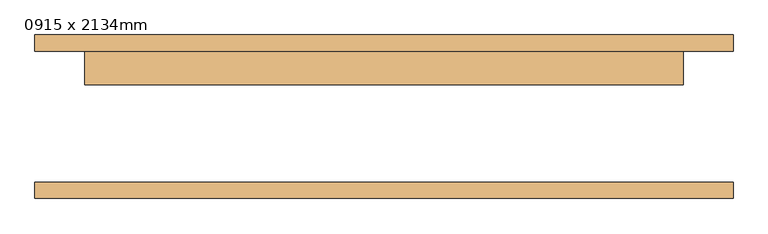
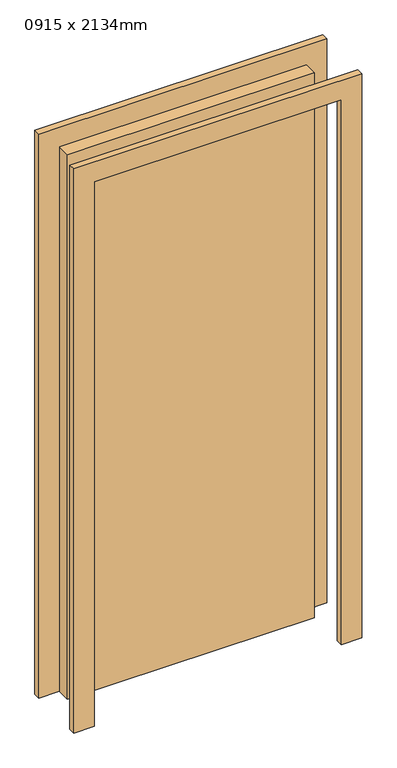
"""IFC4 building model written with IfcOpenShell, lengths in millimetres: door geometry, M_Folha única : 0915 x 2134mm."""

import ifcopenshell
import ifcopenshell.guid

model = None  # the IFC model being written
_history = None  # IfcOwnerHistory: only IFC2X3 demands one
_inside = {}  # id of a spatial element -> (the spatial element, [elements in it])
_under = {}  # id of a project, library or spatial element -> (it, [spatial elements below it])
_declared = {}  # id of a project -> (the project, [libraries it declares])
_typed = {}  # id of a type object -> (the type object, [elements of that type])
_made_of = {}  # id of a material, layer set ... -> (it, [elements and type objects made of it])


def new_model(schema):
    """Start an empty IFC model of exactly this schema.

    Asked for "IFC4X3", IfcOpenShell would pick the latest addendum, in which some entities
    have other attributes; the version numbers below select the first issue.
    IFC2X3 requires an IfcOwnerHistory on every rooted entity: one is made here for all.
    """
    global model, _history
    if schema == "IFC4X3":
        model = ifcopenshell.file(schema_version=(4, 3, 0, 0))
    else:
        model = ifcopenshell.file(schema=schema)
    _inside.clear()
    _under.clear()
    _declared.clear()
    _typed.clear()
    _made_of.clear()
    _history = None
    if model.schema == "IFC2X3":
        org = make("IfcOrganization", Name="unknown")
        user = make(
            "IfcPersonAndOrganization",
            ThePerson=make("IfcPerson", FamilyName="unknown"),
            TheOrganization=org,
        )
        app = make(
            "IfcApplication",
            ApplicationDeveloper=org,
            Version="unknown",
            ApplicationFullName="unknown",
            ApplicationIdentifier="unknown",
        )
        _history = make(
            "IfcOwnerHistory",
            OwningUser=user,
            OwningApplication=app,
            ChangeAction="ADDED",
            CreationDate=0,
        )
    return model


def make(cls, **values):
    """One entity of the class cls with the attributes given. An attribute that is None is left unset."""
    return model.create_entity(
        cls, **{name: value for name, value in values.items() if value is not None}
    )


def rooted(cls, **values):
    """An entity with a GlobalId (a new one), such as an element, a storey or a relation."""
    return make(cls, GlobalId=ifcopenshell.guid.new(), OwnerHistory=_history, **values)


def si_unit(unit_type, name, prefix=None):
    """IfcSIUnit, for example si_unit("LENGTHUNIT", "METRE", prefix="MILLI")."""
    return make("IfcSIUnit", UnitType=unit_type, Prefix=prefix, Name=name)


def assignment(units):
    """IfcUnitAssignment: the units of a project."""
    return None if units is None else make("IfcUnitAssignment", Units=units)


def point(xyz):
    """IfcCartesianPoint."""
    return None if xyz is None else make("IfcCartesianPoint", Coordinates=xyz)


def direction(xyz):
    """IfcDirection."""
    return None if xyz is None else make("IfcDirection", DirectionRatios=xyz)


def frame(location, z_axis=None, x_axis=None):
    """IfcAxis2Placement3D, a coordinate frame: its origin and axes. An axis left out is left unset."""
    return make(
        "IfcAxis2Placement3D",
        Location=point(location),
        Axis=direction(z_axis),
        RefDirection=direction(x_axis),
    )


def origin():
    """The frame at (0, 0, 0) with its axes left unset."""
    return frame((0.0, 0.0, 0.0))


def origin_with_axes():
    """The frame at (0, 0, 0) with the z axis (0, 0, 1) and the x axis (1, 0, 0) written out."""
    return frame((0.0, 0.0, 0.0), z_axis=(0.0, 0.0, 1.0), x_axis=(1.0, 0.0, 0.0))


def place(relative_to, where):
    """IfcLocalPlacement: puts the frame where relative to a parent placement (None: the world)."""
    return make(
        "IfcLocalPlacement", PlacementRelTo=relative_to, RelativePlacement=where
    )


def context(
    kind, dimensions, precision=None, world=None, true_north=None, identifier=None
):
    """IfcGeometricRepresentationContext, for example the 3D "Model" context."""
    return make(
        "IfcGeometricRepresentationContext",
        ContextIdentifier=identifier,
        ContextType=kind,
        CoordinateSpaceDimension=dimensions,
        Precision=precision,
        WorldCoordinateSystem=world,
        TrueNorth=true_north,
    )


def project(units=None, contexts=None):
    """IfcProject with its units and contexts."""
    return rooted(
        "IfcProject",
        Name="project",
        RepresentationContexts=contexts,
        UnitsInContext=assignment(units),
    )


def spatial(cls, under=None, at=None, **own):
    """A site, building, storey or space (cls), placed at a placement, below another one or the project."""
    s = rooted(cls, ObjectPlacement=at, **own)
    if under is not None:
        _under.setdefault(under.id(), (under, []))[1].append(s)
    return s


def polyline(points):
    """IfcPolyline through the points."""
    return make("IfcPolyline", Points=[point(p) for p in points])


def outline(outer, holes=None, kind="AREA"):
    """IfcArbitraryClosedProfileDef: a profile drawn as a closed curve; with holes, ...WithVoids."""
    if holes is None:
        return make("IfcArbitraryClosedProfileDef", ProfileType=kind, OuterCurve=outer)
    return make(
        "IfcArbitraryProfileDefWithVoids",
        ProfileType=kind,
        OuterCurve=outer,
        InnerCurves=holes,
    )


def extrude(swept, where, along, depth):
    """IfcExtrudedAreaSolid: the profile swept, set in the frame where, extruded along a direction by depth."""
    return make(
        "IfcExtrudedAreaSolid",
        SweptArea=swept,
        Position=where,
        ExtrudedDirection=direction(along),
        Depth=depth,
    )


def shape(context_of_items, identifier, shape_type, items):
    """IfcShapeRepresentation: the items that make up one representation, for example the "Body"."""
    return make(
        "IfcShapeRepresentation",
        ContextOfItems=context_of_items,
        RepresentationIdentifier=identifier,
        RepresentationType=shape_type,
        Items=items,
    )


def source(mapping_origin, context_of_items, identifier, shape_type, items):
    """IfcRepresentationMap: a shape defined once, which mapped items show again and again."""
    return make(
        "IfcRepresentationMap",
        MappingOrigin=mapping_origin,
        MappedRepresentation=shape(context_of_items, identifier, shape_type, items),
    )


def transform(
    local_origin,
    x_axis=None,
    y_axis=None,
    z_axis=None,
    scale=None,
    scale2=None,
    scale3=None,
    uniform=True,
):
    """IfcCartesianTransformationOperator3D, or its non-uniform kind. x_axis, y_axis, z_axis: its Axis1, 2, 3."""
    if uniform:
        return make(
            "IfcCartesianTransformationOperator3D",
            Axis1=direction(x_axis),
            Axis2=direction(y_axis),
            LocalOrigin=point(local_origin),
            Scale=scale,
            Axis3=direction(z_axis),
        )
    return make(
        "IfcCartesianTransformationOperator3DnonUniform",
        Axis1=direction(x_axis),
        Axis2=direction(y_axis),
        LocalOrigin=point(local_origin),
        Scale=scale,
        Axis3=direction(z_axis),
        Scale2=scale2,
        Scale3=scale3,
    )


def mapped(mapping_source, mapping_target):
    """IfcMappedItem: shows the shape of a source again, moved by a transform."""
    return make(
        "IfcMappedItem", MappingSource=mapping_source, MappingTarget=mapping_target
    )


def made_of(thing, what):
    """Note that an element or type object is made of a material, layer set ...; save() writes the relation."""
    if what is not None:
        _made_of.setdefault(what.id(), (what, []))[1].append(thing)
    return thing


def element(
    cls,
    number,
    at=None,
    inside=None,
    cuts=None,
    type_object=None,
    material=None,
    context=None,
    identifier="Body",
    shape_type=None,
    held_by="IfcProductDefinitionShape",
    body=None,
    shapes=None,
    **own,
):
    """One element of the class cls, such as IfcWall. Its Tag is "e" and its number.

    at: its placement. inside: the storey or other place that contains it. cuts: it is an
    opening in that element (IfcRelVoidsElement). A single representation is given by context,
    identifier, shape_type and body (its items); several are given by shapes. held_by: the class
    of the entity that holds the representations. save() writes the other relations.
    """
    e = rooted(cls, Tag="e%d" % number, ObjectPlacement=at, **own)
    if body is not None:
        shapes = [shape(context, identifier, shape_type, body)]
    if shapes is not None:
        e.Representation = make(held_by, Representations=shapes)
    if inside is not None:
        _inside.setdefault(inside.id(), (inside, []))[1].append(e)
    if cuts is not None:
        rooted(
            "IfcRelVoidsElement", RelatingBuildingElement=cuts, RelatedOpeningElement=e
        )
    if type_object is not None:
        _typed.setdefault(type_object.id(), (type_object, []))[1].append(e)
    return made_of(e, material)


def aggregate(whole, parts):
    """IfcRelAggregates: a whole, such as a stair, and the parts it consists of."""
    return rooted("IfcRelAggregates", RelatingObject=whole, RelatedObjects=parts)


def save(model, path):
    """Write the relations noted so far, then the file.

    IfcRelAggregates (storeys below a building ...), IfcRelContainedInSpatialStructure (elements
    in a storey), IfcRelDefinesByType, IfcRelAssociatesMaterial and IfcRelDeclares: one each for
    every whole, place, type object, material and project.
    """
    for whole, parts in _under.values():
        aggregate(whole, parts)
    for where, things in _inside.values():
        rooted(
            "IfcRelContainedInSpatialStructure",
            RelatedElements=things,
            RelatingStructure=where,
        )
    for kind, things in _typed.values():
        rooted("IfcRelDefinesByType", RelatedObjects=things, RelatingType=kind)
    for what, things in _made_of.values():
        rooted("IfcRelAssociatesMaterial", RelatedObjects=things, RelatingMaterial=what)
    for by, libraries in _declared.values():
        rooted("IfcRelDeclares", RelatingContext=by, RelatedDefinitions=libraries)
    model.write(path)


def door_0915_x_2134mm_6a9e8738(model_context):
    return source(origin(), model_context, "Body", "SweptSolid", [
        extrude(outline(polyline([(2210.0, -533.5), (0.0, -533.5), (0.0, -457.5), (2134.0, -457.5), (2134.0, 457.5), (0.0, 457.5), (0.0, 533.5), (2210.0, 533.5), (2210.0, -533.5)])), frame((0.0, 100.0, 0.0), z_axis=(0.0, 1.0, 0.0), x_axis=(0.0, 0.0, 1.0)), (0.0, 0.0, 1.0), 25.0),
        extrude(outline(polyline([(2210.0, 533.5), (2210.0, -533.5), (0.0, -533.5), (0.0, -457.5), (2134.0, -457.5), (2134.0, 457.5), (0.0, 457.5), (0.0, 533.5), (2210.0, 533.5)])), frame((0.0, -125.0, 0.0), z_axis=(0.0, 1.0, 0.0), x_axis=(0.0, 0.0, 1.0)), (0.0, 0.0, 1.0), 25.0),
        extrude(outline(polyline([(457.5, 49.0), (-457.5, 49.0), (-457.5, 100.0), (457.5, 100.0), (457.5, 49.0)])), origin_with_axes(), (0.0, 0.0, 1.0), 2134.0),
    ])


if __name__ == "__main__":
    model = new_model("IFC4")
    model_context = context("Model", 3, world=origin())
    ifc_project = project(units=[si_unit("LENGTHUNIT", "METRE", prefix="MILLI")], contexts=[model_context])
    site = spatial("IfcSite", under=ifc_project)
    building = spatial("IfcBuilding", under=site)
    placement = place(None, origin())
    door_0915_x_2134mm_shape = door_0915_x_2134mm_6a9e8738(model_context)
    element("IfcDoor", 1, ObjectType="M_Folha única : 0915 x 2134mm", at=placement, inside=building, context=model_context, shape_type="MappedRepresentation", body=[
        mapped(door_0915_x_2134mm_shape, transform((0.0, 0.0, 0.0), x_axis=(1.0, 0.0, 0.0), y_axis=(0.0, 1.0, 0.0), z_axis=(0.0, 0.0, 1.0))),
    ])
    save(model, "model.ifc")

# Revit data of these elements
# Project information
#   Data de emissão do projeto = "Data de emissão"
#   Status do projeto = "Status do projeto"
#   Nome do cliente = "Proprietário"
#   Endereço do projeto = "Insira aqui o endereço"
#   Nome do projeto = "Nome do projeto"
#   Número do projeto = "0001"
# Type "M_Folha única : 0915 x 2134mm"
#   Type Mark = "20"
#   Construction Type Id = "MDOOR"
#   Analytic Construction = "Metal"
#   Thickness = 0.051 m
#   Thermal Resistance (R) = 0.270117 (m²·K)/W
#   Heat Transfer Coefficient (U) = 3.7021 W/(m²·K)
#   Height = 2.134 m
#   Projeção da apara externa = 0.025 m
#   Projeção da apara interna = 0.025 m
#   Largura da apara = 0.076 m
#   Width = 0.915 m
#   Define Thermal Properties by = 1
#   Define Thermal Properties by = 1
#   Material da porta = Porta - Painel
#   Material da moldura = Porta - Batente
#   Visual Light Transmittance = 0
#   Solar Heat Gain Coefficient = 0
#   Function = (empty or 0)
#   Wall Closure = (empty or 0)
# Element 1 (IfcDoor, "M_Folha única : 0915 x 2134mm")
#   Materials on its faces: "Porta - Batente", "Porta - Painel"
# Materials
#   "Porta - Painel": class "Madeira", colour RGB 210 159 95, transparency 0, Cost = 0
#   "Porta - Batente": class "Diversos", colour RGB 118 70 51, transparency 0, Cost = 0
